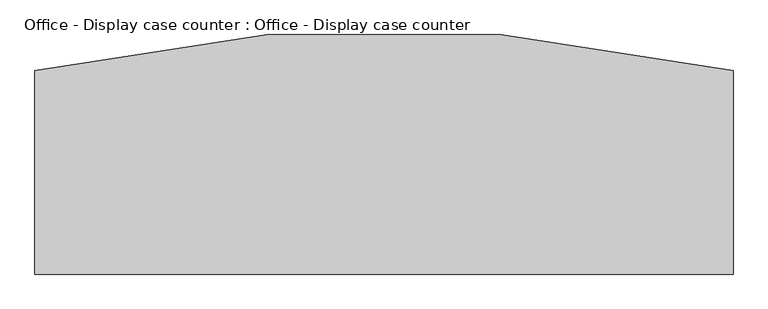
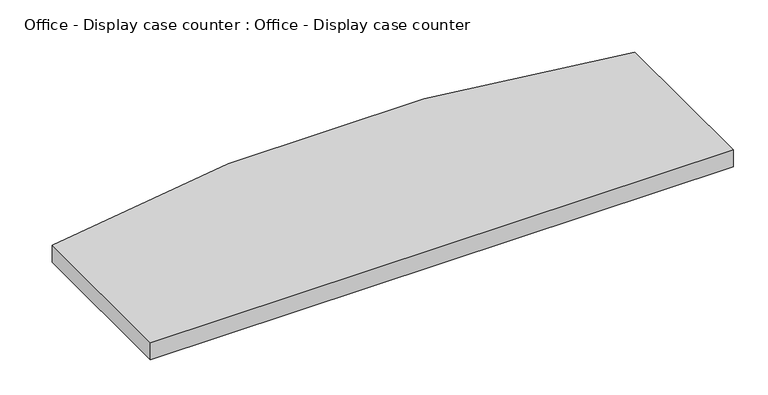
"""IFC4 building model written with IfcOpenShell, lengths in millimetres: furniture geometry, Office - Display case counter : Office - Display case counter."""

from ifc_helpers import new_model, si_unit, point, frame, frame_2d, origin, place, context, project, spatial, polyline, circle_curve, trimmed, segment, composite_curve, outline, extrude, source, transform, mapped, element, save


def office_display_case_counter_office_display_case_counter_2949f9fd(model_context):
    return source(origin(), model_context, "Body", "SweptSolid", [
        extrude(outline(composite_curve([segment(polyline([(-4564.0279916, 13394.6070453), (-4564.0279916, 13750.2070453)]), True, "CONTINUOUS"), segment(trimmed(circle_curve(frame_2d((-3954.4279916, 11157.1726729)), 2663.7266032), [point((-4564.0279916, 13750.2070453))], [point((-3344.8279916, 13750.2070453))], False, "CARTESIAN"), True, "CONTINUOUS"), segment(polyline([(-3344.8279916, 13750.2070453), (-3344.8279916, 13394.6070453), (-4564.0279916, 13394.6070453)]), True, "CONTINUOUS")], self_intersect=False)), frame((0.0, 0.0, 876.3), z_axis=(0.0, 0.0, 1.0), x_axis=(1.0, 0.0, 0.0)), (0.0, 0.0, 1.0), 38.1),
    ])


if __name__ == "__main__":
    model = new_model("IFC4")
    model_context = context("Model", 3, world=origin())
    ifc_project = project(units=[si_unit("LENGTHUNIT", "METRE", prefix="MILLI")], contexts=[model_context])
    site = spatial("IfcSite", under=ifc_project)
    building = spatial("IfcBuilding", under=site)
    placement = place(None, origin())
    office_display_case_counter_office_display_case_counter_shape = office_display_case_counter_office_display_case_counter_2949f9fd(model_context)
    element("IfcFurniture", 1, ObjectType="Office - Display case counter : Office - Display case counter", at=placement, inside=building, context=model_context, shape_type="MappedRepresentation", body=[
        mapped(office_display_case_counter_office_display_case_counter_shape, transform((0.0, 0.0, 0.0), x_axis=(1.0, 0.0, 0.0), y_axis=(0.0, 1.0, 0.0), z_axis=(0.0, 0.0, 1.0))),
    ])
    save(model, "model.ifc")

# Revit data of these elements
# Type "Office - Display case counter : Office - Display case counter"
#   COBie.Type = no
# Element 1 (IfcFurniture, "Office - Display case counter : Office - Display case counter")
#   Materials on its faces: "Green Laminate"
# Materials
#   "Green Laminate": class "Generic", colour RGB 57 96 54, transparency 0, Cost = 0
